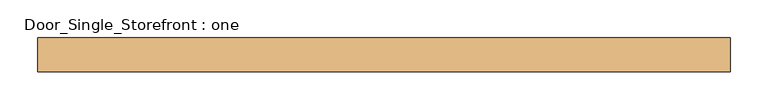
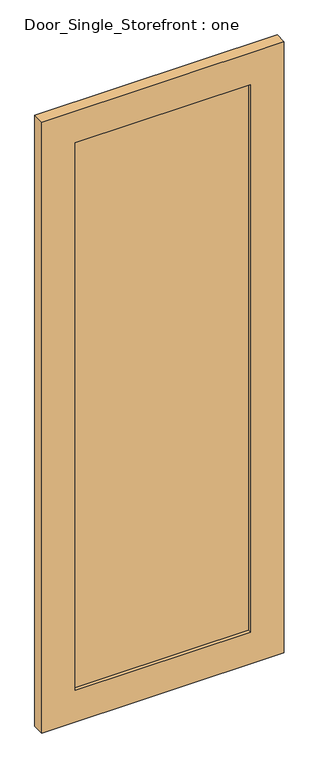
"""IFC4 building model written with IfcOpenShell, lengths in millimetres: door geometry, Door_Single_Storefront : one."""

from ifc_helpers import new_model, si_unit, frame, origin, place, context, project, spatial, polyline, outline, extrude, source, transform, mapped, element, save


def door_single_storefront_one_661f645a(model_context):
    return source(origin(), model_context, "Body", "SweptSolid", [
        extrude(outline(polyline([(330.2, -6.35), (-330.2, -6.35), (-330.2, 12.7), (330.2, 12.7), (330.2, -6.35)])), frame((0.0, 0.0, 127.0), z_axis=(0.0, 0.0, 1.0), x_axis=(1.0, 0.0, 0.0)), (0.0, 0.0, 1.0), 2180.3688887),
        extrude(outline(polyline([(2434.3688887, -457.2), (0.0, -457.2), (0.0, 457.2), (2434.3688887, 457.2), (2434.3688887, -457.2)]), holes=[polyline([(127.0, 330.2), (127.0, -330.2), (2307.3688887, -330.2), (2307.3688887, 330.2), (127.0, 330.2)])]), frame((0.0, -19.05, 0.0), z_axis=(0.0, 1.0, 0.0), x_axis=(0.0, 0.0, 1.0)), (0.0, 0.0, 1.0), 44.45),
    ])


if __name__ == "__main__":
    model = new_model("IFC4")
    model_context = context("Model", 3, world=origin())
    ifc_project = project(units=[si_unit("LENGTHUNIT", "METRE", prefix="MILLI")], contexts=[model_context])
    site = spatial("IfcSite", under=ifc_project)
    building = spatial("IfcBuilding", under=site)
    placement = place(None, origin())
    door_single_storefront_one_shape = door_single_storefront_one_661f645a(model_context)
    element("IfcDoor", 1, ObjectType="Door_Single_Storefront : one", at=placement, inside=building, context=model_context, shape_type="MappedRepresentation", body=[
        mapped(door_single_storefront_one_shape, transform((0.0, 0.0, 0.0), x_axis=(1.0, 0.0, 0.0), y_axis=(0.0, 1.0, 0.0), z_axis=(0.0, 0.0, 1.0))),
    ])
    save(model, "model.ifc")

# Revit data of these elements
# Type "Door_Single_Storefront : one"
#   Type Mark = "29"
#   Analytic Construction = "<None>"
#   Stile_Width = 0' - 5"
#   Door_Thickness = 0' - 1 3/4"
#   Door_Offset = 0' - 1"
#   Glass_Material = INSULATED GLAZING
#   Frame_Material = ALUMINUM STOREFRONT
#   Function = (empty or 0)
# Element 1 (IfcDoor, "Door_Single_Storefront : one")
#   Materials on its faces: "ALUMINUM STOREFRONT", "INSULATED GLAZING"
# Materials
#   "INSULATED GLAZING": class "Glass", colour RGB 196 205 210, transparency 0.85, Description = "Soda Lime Glass", Cost = 0
#   "ALUMINUM STOREFRONT": class "Metal", colour RGB 244 244 244, transparency 0, Description = "Aluminum 6061", Cost = 0
